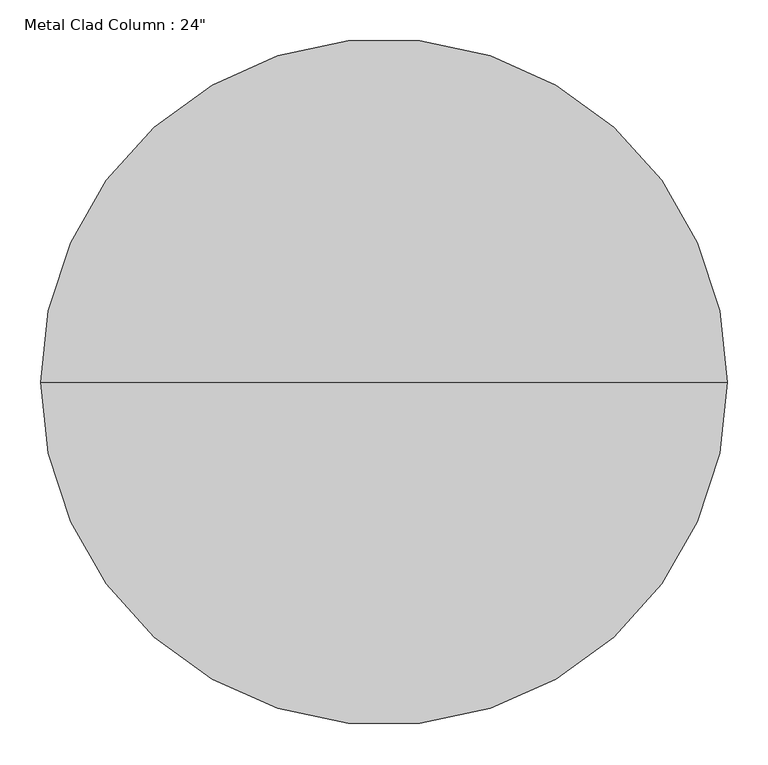
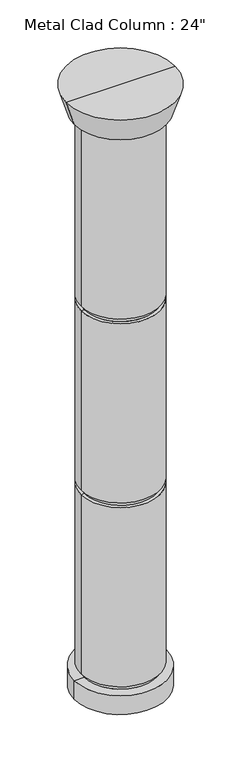
"""IFC4 building model written with IfcOpenShell, lengths in millimetres: column geometry."""

from ifc_helpers import new_model, si_unit, frame, origin, place, context, project, spatial, polyline, circle_curve, source, transform, mapped, element, save
from ifc_brep_helpers import plane_surface, cylinder_surface, revolved_surface, advanced_brep


def column_9238a582(model_context):
    return source(origin(), model_context, "Body", "AdvancedBrep", [
        advanced_brep(
        [(0.0, 0.0, 0.0), (-355.6, 0.0, 0.0), (355.6, 0.0, 0.0), (-355.6, 0.0, 152.4), (355.6, 0.0, 152.4), (279.4, 0.0, 1684.8666667), (-279.4, 0.0, 1684.8666667), (-304.8, 0.0, 1684.8666667), (304.8, 0.0, 1684.8666667), (-304.8, 0.0, 3141.1333333), (304.8, 0.0, 3141.1333333), (279.4, 0.0, 1646.7666667), (-279.4, 0.0, 1646.7666667), (304.8, 0.0, 1646.7666667), (-304.8, 0.0, 1646.7666667), (304.8, 0.0, 190.5), (-304.8, 0.0, 190.5), (279.4, 0.0, 190.5), (-279.4, 0.0, 190.5), (279.4, 0.0, 152.4), (-279.4, 0.0, 152.4), (355.6, 0.0, 4673.6), (-355.6, 0.0, 4673.6), (-419.1, 0.0, 4876.8), (419.1, 0.0, 4876.8), (0.0, 0.0, 4876.8), (279.4, 0.0, 4673.6), (-279.4, 0.0, 4673.6), (279.4, 0.0, 4635.5), (-279.4, 0.0, 4635.5), (304.8, 0.0, 4635.5), (-304.8, 0.0, 4635.5), (304.8, 0.0, 3179.2333333), (-304.8, 0.0, 3179.2333333), (279.4, 0.0, 3179.2333333), (-279.4, 0.0, 3179.2333333), (279.4, 0.0, 3141.1333333), (-279.4, 0.0, 3141.1333333)],
        [
            (0, 1),
            (1, 2, circle_curve(frame((0.0, 0.0, 0.0), z_axis=(0.0, 0.0, -1.0), x_axis=(-1.0, 0.0, 0.0)), 355.6)),
            (2, 0),
            (2, 1, circle_curve(frame((0.0, 0.0, 0.0), z_axis=(0.0, 0.0, -1.0), x_axis=(-1.0, 0.0, 0.0)), 355.6)),
            (1, 3),
            (3, 4, circle_curve(frame((0.0, 0.0, 152.4), z_axis=(0.0, 0.0, -1.0), x_axis=(-1.0, 0.0, 0.0)), 355.6)),
            (4, 2),
            (4, 3, circle_curve(frame((0.0, 0.0, 152.4), z_axis=(0.0, 0.0, -1.0), x_axis=(-1.0, 0.0, 0.0)), 355.6)),
            (5, 6, circle_curve(frame((0.0, 0.0, 1684.8666667), z_axis=(0.0, 0.0, 1.0), x_axis=(-1.0, 0.0, 0.0)), 279.4)),
            (6, 7),
            (7, 8, circle_curve(frame((0.0, 0.0, 1684.8666667), z_axis=(0.0, 0.0, -1.0), x_axis=(-1.0, 0.0, 0.0)), 304.8)),
            (8, 5),
            (7, 9),
            (9, 10, circle_curve(frame((0.0, 0.0, 3141.1333333), z_axis=(0.0, 0.0, -1.0), x_axis=(-1.0, 0.0, 0.0)), 304.8)),
            (10, 8),
            (7, 8, circle_curve(frame((0.0, 0.0, 1684.8666667), z_axis=(0.0, 0.0, 1.0), x_axis=(-1.0, 0.0, 0.0)), 304.8)),
            (10, 9, circle_curve(frame((0.0, 0.0, 3141.1333333), z_axis=(0.0, 0.0, -1.0), x_axis=(-1.0, 0.0, 0.0)), 304.8)),
            (6, 5, circle_curve(frame((0.0, 0.0, 1684.8666667), z_axis=(0.0, 0.0, 1.0), x_axis=(-1.0, 0.0, 0.0)), 279.4)),
            (11, 12, circle_curve(frame((0.0, 0.0, 1646.7666667), z_axis=(0.0, 0.0, 1.0), x_axis=(-1.0, 0.0, 0.0)), 279.4)),
            (12, 6),
            (5, 11),
            (12, 11, circle_curve(frame((0.0, 0.0, 1646.7666667), z_axis=(0.0, 0.0, 1.0), x_axis=(-1.0, 0.0, 0.0)), 279.4)),
            (13, 14, circle_curve(frame((0.0, 0.0, 1646.7666667), z_axis=(0.0, 0.0, 1.0), x_axis=(-1.0, 0.0, 0.0)), 304.8)),
            (14, 12),
            (11, 13),
            (14, 13, circle_curve(frame((0.0, 0.0, 1646.7666667), z_axis=(0.0, 0.0, 1.0), x_axis=(-1.0, 0.0, 0.0)), 304.8)),
            (15, 16, circle_curve(frame((0.0, 0.0, 190.5), z_axis=(0.0, 0.0, 1.0), x_axis=(-1.0, 0.0, 0.0)), 304.8)),
            (16, 14),
            (13, 15),
            (16, 15, circle_curve(frame((0.0, 0.0, 190.5), z_axis=(0.0, 0.0, 1.0), x_axis=(-1.0, 0.0, 0.0)), 304.8)),
            (17, 18, circle_curve(frame((0.0, 0.0, 190.5), z_axis=(0.0, 0.0, 1.0), x_axis=(-1.0, 0.0, 0.0)), 279.4)),
            (18, 16),
            (15, 17),
            (18, 17, circle_curve(frame((0.0, 0.0, 190.5), z_axis=(0.0, 0.0, 1.0), x_axis=(-1.0, 0.0, 0.0)), 279.4)),
            (19, 20, circle_curve(frame((0.0, 0.0, 152.4), z_axis=(0.0, 0.0, 1.0), x_axis=(-1.0, 0.0, 0.0)), 279.4)),
            (20, 18),
            (17, 19),
            (20, 19, circle_curve(frame((0.0, 0.0, 152.4), z_axis=(0.0, 0.0, 1.0), x_axis=(-1.0, 0.0, 0.0)), 279.4)),
            (3, 20),
            (19, 4),
            (21, 22, circle_curve(frame((0.0, 0.0, 4673.6), z_axis=(0.0, 0.0, 1.0), x_axis=(-1.0, 0.0, 0.0)), 355.6)),
            (22, 23),
            (23, 24, circle_curve(frame((0.0, 0.0, 4876.8), z_axis=(0.0, 0.0, -1.0), x_axis=(-1.0, 0.0, 0.0)), 419.1)),
            (24, 21),
            (23, 25),
            (25, 24),
            (23, 24, circle_curve(frame((0.0, 0.0, 4876.8), z_axis=(0.0, 0.0, 1.0), x_axis=(-1.0, 0.0, 0.0)), 419.1)),
            (22, 21, circle_curve(frame((0.0, 0.0, 4673.6), z_axis=(0.0, 0.0, 1.0), x_axis=(-1.0, 0.0, 0.0)), 355.6)),
            (26, 27, circle_curve(frame((0.0, 0.0, 4673.6), z_axis=(0.0, 0.0, 1.0), x_axis=(-1.0, 0.0, 0.0)), 279.4)),
            (27, 22),
            (21, 26),
            (27, 26, circle_curve(frame((0.0, 0.0, 4673.6), z_axis=(0.0, 0.0, 1.0), x_axis=(-1.0, 0.0, 0.0)), 279.4)),
            (28, 29, circle_curve(frame((0.0, 0.0, 4635.5), z_axis=(0.0, 0.0, 1.0), x_axis=(-1.0, 0.0, 0.0)), 279.4)),
            (29, 27),
            (26, 28),
            (29, 28, circle_curve(frame((0.0, 0.0, 4635.5), z_axis=(0.0, 0.0, 1.0), x_axis=(-1.0, 0.0, 0.0)), 279.4)),
            (30, 31, circle_curve(frame((0.0, 0.0, 4635.5), z_axis=(0.0, 0.0, 1.0), x_axis=(-1.0, 0.0, 0.0)), 304.8)),
            (31, 29),
            (28, 30),
            (31, 30, circle_curve(frame((0.0, 0.0, 4635.5), z_axis=(0.0, 0.0, 1.0), x_axis=(-1.0, 0.0, 0.0)), 304.8)),
            (32, 33, circle_curve(frame((0.0, 0.0, 3179.2333333), z_axis=(0.0, 0.0, 1.0), x_axis=(-1.0, 0.0, 0.0)), 304.8)),
            (33, 31),
            (30, 32),
            (33, 32, circle_curve(frame((0.0, 0.0, 3179.2333333), z_axis=(0.0, 0.0, 1.0), x_axis=(-1.0, 0.0, 0.0)), 304.8)),
            (34, 35, circle_curve(frame((0.0, 0.0, 3179.2333333), z_axis=(0.0, 0.0, 1.0), x_axis=(-1.0, 0.0, 0.0)), 279.4)),
            (35, 33),
            (32, 34),
            (35, 34, circle_curve(frame((0.0, 0.0, 3179.2333333), z_axis=(0.0, 0.0, 1.0), x_axis=(-1.0, 0.0, 0.0)), 279.4)),
            (36, 37, circle_curve(frame((0.0, 0.0, 3141.1333333), z_axis=(0.0, 0.0, 1.0), x_axis=(-1.0, 0.0, 0.0)), 279.4)),
            (37, 35),
            (34, 36),
            (37, 36, circle_curve(frame((0.0, 0.0, 3141.1333333), z_axis=(0.0, 0.0, 1.0), x_axis=(-1.0, 0.0, 0.0)), 279.4)),
            (9, 37),
            (36, 10),
        ],
        [
            plane_surface(frame((0.0, 0.0, 0.0), z_axis=(0.0, 0.0, -1.0), x_axis=(-1.0, 0.0, 0.0))),
            cylinder_surface(frame((0.0, 0.0, 4876.8), z_axis=(0.0, 0.0, -1.0), x_axis=(-1.0, 0.0, 0.0)), 355.6),
            plane_surface(frame((0.0, 0.0, 1684.8666667), z_axis=(0.0, 0.0, -1.0), x_axis=(-1.0, 0.0, 0.0))),
            cylinder_surface(frame((0.0, 0.0, 4876.8), z_axis=(0.0, 0.0, -1.0), x_axis=(-1.0, 0.0, 0.0)), 304.8),
            cylinder_surface(frame((0.0, 0.0, 4876.8), z_axis=(0.0, 0.0, -1.0), x_axis=(-1.0, 0.0, 0.0)), 279.4),
            plane_surface(frame((0.0, 0.0, 1646.7666667), z_axis=(0.0, 0.0, 1.0), x_axis=(-1.0, 0.0, 0.0))),
            plane_surface(frame((0.0, 0.0, 190.5), z_axis=(0.0, 0.0, -1.0), x_axis=(-1.0, 0.0, 0.0))),
            plane_surface(frame((0.0, 0.0, 152.4), z_axis=(0.0, 0.0, 1.0), x_axis=(-1.0, 0.0, 0.0))),
            revolved_surface(polyline([(-419.1, 0.0, 4876.8), (-355.6, 0.0, 4673.6)]), (0.0, 0.0, 4876.8), (0.0, 0.0, -1.0)),
            plane_surface(frame((0.0, 0.0, 4876.8), z_axis=(0.0, 0.0, 1.0), x_axis=(-1.0, 0.0, 0.0))),
            plane_surface(frame((0.0, 0.0, 4673.6), z_axis=(0.0, 0.0, -1.0), x_axis=(-1.0, 0.0, 0.0))),
            plane_surface(frame((0.0, 0.0, 4635.5), z_axis=(0.0, 0.0, 1.0), x_axis=(-1.0, 0.0, 0.0))),
            plane_surface(frame((0.0, 0.0, 3179.2333333), z_axis=(0.0, 0.0, -1.0), x_axis=(-1.0, 0.0, 0.0))),
            plane_surface(frame((0.0, 0.0, 3141.1333333), z_axis=(0.0, 0.0, 1.0), x_axis=(-1.0, 0.0, 0.0))),
        ],
        [
            (0, [[1, 2, 3]]),
            (0, [[-3, 4, -1]]),
            (1, [[-2, 5, 6, 7]]),
            (1, [[-4, -7, 8, -5]]),
            (2, [[9, 10, 11, 12]]),
            (3, [[-11, 13, 14, 15]]),
            (3, [[16, -15, 17, -13]]),
            (2, [[18, -12, -16, -10]]),
            (4, [[19, 20, -9, 21]]),
            (4, [[22, -21, -18, -20]]),
            (5, [[23, 24, -19, 25]]),
            (5, [[26, -25, -22, -24]]),
            (3, [[27, 28, -23, 29]]),
            (3, [[30, -29, -26, -28]]),
            (6, [[31, 32, -27, 33]]),
            (6, [[34, -33, -30, -32]]),
            (4, [[35, 36, -31, 37]]),
            (4, [[38, -37, -34, -36]]),
            (7, [[-6, 39, -35, 40]]),
            (7, [[-8, -40, -38, -39]]),
            (8, [[41, 42, 43, 44]]),
            (9, [[-43, 45, 46]]),
            (9, [[47, -46, -45]]),
            (8, [[48, -44, -47, -42]]),
            (10, [[49, 50, -41, 51]]),
            (10, [[52, -51, -48, -50]]),
            (4, [[53, 54, -49, 55]]),
            (4, [[56, -55, -52, -54]]),
            (11, [[57, 58, -53, 59]]),
            (11, [[60, -59, -56, -58]]),
            (3, [[61, 62, -57, 63]]),
            (3, [[64, -63, -60, -62]]),
            (12, [[65, 66, -61, 67]]),
            (12, [[68, -67, -64, -66]]),
            (4, [[69, 70, -65, 71]]),
            (4, [[72, -71, -68, -70]]),
            (13, [[-14, 73, -69, 74]]),
            (13, [[-17, -74, -72, -73]]),
        ],
    ),
    ])


if __name__ == "__main__":
    model = new_model("IFC4")
    model_context = context("Model", 3, world=origin())
    ifc_project = project(units=[si_unit("LENGTHUNIT", "METRE", prefix="MILLI")], contexts=[model_context])
    site = spatial("IfcSite", under=ifc_project)
    building = spatial("IfcBuilding", under=site)
    placement = place(None, origin())
    column_shape = column_9238a582(model_context)
    element("IfcColumn", 1, ObjectType="Metal Clad Column : 24\"", at=placement, inside=building, context=model_context, shape_type="MappedRepresentation", body=[
        mapped(column_shape, transform((0.0, 0.0, 0.0), x_axis=(1.0, 0.0, 0.0), y_axis=(0.0, 1.0, 0.0), z_axis=(0.0, 0.0, 1.0))),
    ])
    save(model, "model.ifc")

# Revit data of these elements
# Type "Metal Clad Column : 24\""
#   Assembly Code = "B1010200"
#   Base = 0' - 6"
#   Capital = 0' - 8"
#   Diameter = 2' - 0"
#   Joint Depth = 0' - 1"
#   Joint Width = 0' - 1 1/2"
#   Offset base level = 0' - 0"
#   Offset top level = 0' - 0"
#   Material = Aluminum
# Element 1 (IfcColumn, "Metal Clad Column : 24\"")
#   Materials on its faces: "Aluminum"
# Materials
#   "Aluminum": class "Metal", colour RGB 247 247 247, transparency 0, Description = "Aluminum 6061", Cost = 0
